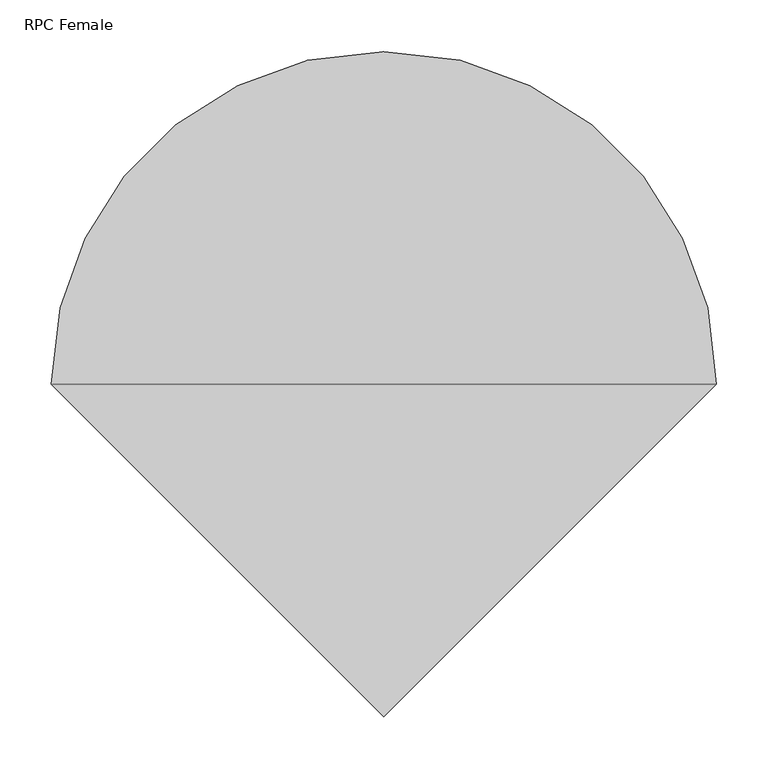
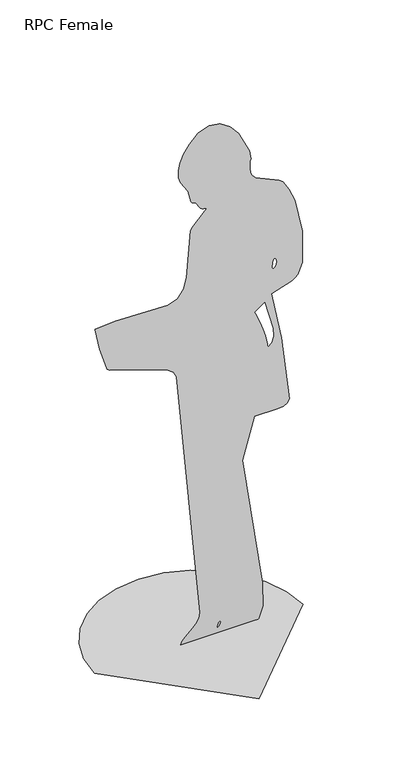
"""IFC4 building model written with IfcOpenShell, lengths in millimetres: proxy geometry, RPC Female : Lisa."""

import ifcopenshell
import ifcopenshell.guid

model = None  # the IFC model being written
_history = None  # IfcOwnerHistory: only IFC2X3 demands one
_inside = {}  # id of a spatial element -> (the spatial element, [elements in it])
_under = {}  # id of a project, library or spatial element -> (it, [spatial elements below it])
_declared = {}  # id of a project -> (the project, [libraries it declares])
_typed = {}  # id of a type object -> (the type object, [elements of that type])
_made_of = {}  # id of a material, layer set ... -> (it, [elements and type objects made of it])


def new_model(schema):
    """Start an empty IFC model of exactly this schema.

    Asked for "IFC4X3", IfcOpenShell would pick the latest addendum, in which some entities
    have other attributes; the version numbers below select the first issue.
    IFC2X3 requires an IfcOwnerHistory on every rooted entity: one is made here for all.
    """
    global model, _history
    if schema == "IFC4X3":
        model = ifcopenshell.file(schema_version=(4, 3, 0, 0))
    else:
        model = ifcopenshell.file(schema=schema)
    _inside.clear()
    _under.clear()
    _declared.clear()
    _typed.clear()
    _made_of.clear()
    _history = None
    if model.schema == "IFC2X3":
        org = make("IfcOrganization", Name="unknown")
        user = make(
            "IfcPersonAndOrganization",
            ThePerson=make("IfcPerson", FamilyName="unknown"),
            TheOrganization=org,
        )
        app = make(
            "IfcApplication",
            ApplicationDeveloper=org,
            Version="unknown",
            ApplicationFullName="unknown",
            ApplicationIdentifier="unknown",
        )
        _history = make(
            "IfcOwnerHistory",
            OwningUser=user,
            OwningApplication=app,
            ChangeAction="ADDED",
            CreationDate=0,
        )
    return model


def make(cls, **values):
    """One entity of the class cls with the attributes given. An attribute that is None is left unset."""
    return model.create_entity(
        cls, **{name: value for name, value in values.items() if value is not None}
    )


def rooted(cls, **values):
    """An entity with a GlobalId (a new one), such as an element, a storey or a relation."""
    return make(cls, GlobalId=ifcopenshell.guid.new(), OwnerHistory=_history, **values)


def si_unit(unit_type, name, prefix=None):
    """IfcSIUnit, for example si_unit("LENGTHUNIT", "METRE", prefix="MILLI")."""
    return make("IfcSIUnit", UnitType=unit_type, Prefix=prefix, Name=name)


def assignment(units):
    """IfcUnitAssignment: the units of a project."""
    return None if units is None else make("IfcUnitAssignment", Units=units)


def point(xyz):
    """IfcCartesianPoint."""
    return None if xyz is None else make("IfcCartesianPoint", Coordinates=xyz)


def direction(xyz):
    """IfcDirection."""
    return None if xyz is None else make("IfcDirection", DirectionRatios=xyz)


def frame(location, z_axis=None, x_axis=None):
    """IfcAxis2Placement3D, a coordinate frame: its origin and axes. An axis left out is left unset."""
    return make(
        "IfcAxis2Placement3D",
        Location=point(location),
        Axis=direction(z_axis),
        RefDirection=direction(x_axis),
    )


def origin():
    """The frame at (0, 0, 0) with its axes left unset."""
    return frame((0.0, 0.0, 0.0))


def place(relative_to, where):
    """IfcLocalPlacement: puts the frame where relative to a parent placement (None: the world)."""
    return make(
        "IfcLocalPlacement", PlacementRelTo=relative_to, RelativePlacement=where
    )


def context(
    kind, dimensions, precision=None, world=None, true_north=None, identifier=None
):
    """IfcGeometricRepresentationContext, for example the 3D "Model" context."""
    return make(
        "IfcGeometricRepresentationContext",
        ContextIdentifier=identifier,
        ContextType=kind,
        CoordinateSpaceDimension=dimensions,
        Precision=precision,
        WorldCoordinateSystem=world,
        TrueNorth=true_north,
    )


def project(units=None, contexts=None):
    """IfcProject with its units and contexts."""
    return rooted(
        "IfcProject",
        Name="project",
        RepresentationContexts=contexts,
        UnitsInContext=assignment(units),
    )


def spatial(cls, under=None, at=None, **own):
    """A site, building, storey or space (cls), placed at a placement, below another one or the project."""
    s = rooted(cls, ObjectPlacement=at, **own)
    if under is not None:
        _under.setdefault(under.id(), (under, []))[1].append(s)
    return s


def point_list(points):
    """IfcCartesianPointList2D or 3D."""
    cls = (
        "IfcCartesianPointList2D" if len(points[0]) == 2 else "IfcCartesianPointList3D"
    )
    return make(cls, CoordList=points)


def triangles(points, corners, closed=None, point_numbers=None):
    """IfcTriangulatedFaceSet: each triangle names its three corners, points numbered from 1."""
    return make(
        "IfcTriangulatedFaceSet",
        Coordinates=point_list(points),
        Closed=closed,
        CoordIndex=corners,
        PnIndex=point_numbers,
    )


def shape(context_of_items, identifier, shape_type, items):
    """IfcShapeRepresentation: the items that make up one representation, for example the "Body"."""
    return make(
        "IfcShapeRepresentation",
        ContextOfItems=context_of_items,
        RepresentationIdentifier=identifier,
        RepresentationType=shape_type,
        Items=items,
    )


def source(mapping_origin, context_of_items, identifier, shape_type, items):
    """IfcRepresentationMap: a shape defined once, which mapped items show again and again."""
    return make(
        "IfcRepresentationMap",
        MappingOrigin=mapping_origin,
        MappedRepresentation=shape(context_of_items, identifier, shape_type, items),
    )


def transform(
    local_origin,
    x_axis=None,
    y_axis=None,
    z_axis=None,
    scale=None,
    scale2=None,
    scale3=None,
    uniform=True,
):
    """IfcCartesianTransformationOperator3D, or its non-uniform kind. x_axis, y_axis, z_axis: its Axis1, 2, 3."""
    if uniform:
        return make(
            "IfcCartesianTransformationOperator3D",
            Axis1=direction(x_axis),
            Axis2=direction(y_axis),
            LocalOrigin=point(local_origin),
            Scale=scale,
            Axis3=direction(z_axis),
        )
    return make(
        "IfcCartesianTransformationOperator3DnonUniform",
        Axis1=direction(x_axis),
        Axis2=direction(y_axis),
        LocalOrigin=point(local_origin),
        Scale=scale,
        Axis3=direction(z_axis),
        Scale2=scale2,
        Scale3=scale3,
    )


def mapped(mapping_source, mapping_target):
    """IfcMappedItem: shows the shape of a source again, moved by a transform."""
    return make(
        "IfcMappedItem", MappingSource=mapping_source, MappingTarget=mapping_target
    )


def made_of(thing, what):
    """Note that an element or type object is made of a material, layer set ...; save() writes the relation."""
    if what is not None:
        _made_of.setdefault(what.id(), (what, []))[1].append(thing)
    return thing


def element(
    cls,
    number,
    at=None,
    inside=None,
    cuts=None,
    type_object=None,
    material=None,
    context=None,
    identifier="Body",
    shape_type=None,
    held_by="IfcProductDefinitionShape",
    body=None,
    shapes=None,
    **own,
):
    """One element of the class cls, such as IfcWall. Its Tag is "e" and its number.

    at: its placement. inside: the storey or other place that contains it. cuts: it is an
    opening in that element (IfcRelVoidsElement). A single representation is given by context,
    identifier, shape_type and body (its items); several are given by shapes. held_by: the class
    of the entity that holds the representations. save() writes the other relations.
    """
    e = rooted(cls, Tag="e%d" % number, ObjectPlacement=at, **own)
    if body is not None:
        shapes = [shape(context, identifier, shape_type, body)]
    if shapes is not None:
        e.Representation = make(held_by, Representations=shapes)
    if inside is not None:
        _inside.setdefault(inside.id(), (inside, []))[1].append(e)
    if cuts is not None:
        rooted(
            "IfcRelVoidsElement", RelatingBuildingElement=cuts, RelatedOpeningElement=e
        )
    if type_object is not None:
        _typed.setdefault(type_object.id(), (type_object, []))[1].append(e)
    return made_of(e, material)


def aggregate(whole, parts):
    """IfcRelAggregates: a whole, such as a stair, and the parts it consists of."""
    return rooted("IfcRelAggregates", RelatingObject=whole, RelatedObjects=parts)


def save(model, path):
    """Write the relations noted so far, then the file.

    IfcRelAggregates (storeys below a building ...), IfcRelContainedInSpatialStructure (elements
    in a storey), IfcRelDefinesByType, IfcRelAssociatesMaterial and IfcRelDeclares: one each for
    every whole, place, type object, material and project.
    """
    for whole, parts in _under.values():
        aggregate(whole, parts)
    for where, things in _inside.values():
        rooted(
            "IfcRelContainedInSpatialStructure",
            RelatedElements=things,
            RelatingStructure=where,
        )
    for kind, things in _typed.values():
        rooted("IfcRelDefinesByType", RelatedObjects=things, RelatingType=kind)
    for what, things in _made_of.values():
        rooted("IfcRelAssociatesMaterial", RelatedObjects=things, RelatingMaterial=what)
    for by, libraries in _declared.values():
        rooted("IfcRelDeclares", RelatingContext=by, RelatedDefinitions=libraries)
    model.write(path)


def rpc_female_aec5a013(model_context):
    return source(origin(), model_context, "Body", "Tessellation", [
        triangles([(323.55714, 0.0002011, 4.31e-05), (315.003338, 74.1380801, 4.31e-05), (290.6422523, 142.2218604, 4.31e-05), (252.4244724, 202.3008604, 4.31e-05), (202.3008059, 252.4245814, 4.31e-05), (142.2217514, 290.6422886, 4.31e-05), (74.1379711, 315.003447, 4.31e-05), (0.0001118, 323.557249, 4.31e-05), (-74.1377576, 315.003447, 4.31e-05), (-142.2215424, 290.6423431, 4.31e-05), (-202.3005515, 252.4245814, 4.31e-05), (-252.4243089, 202.3009149, 4.31e-05), (-290.6419797, 142.2218422, 4.31e-05), (-315.0031199, 74.1380664, 4.31e-05), (-323.556922, 0.0002066, 4.31e-05), (0.0001345, -323.556813, 4.31e-05), (239.7155461, -0.0024821, 1166.2291054), (241.5671591, -0.0024453, 1161.6157969), (242.5844117, -0.0023971, 1155.5697269), (242.4387992, -0.0023449, 1149.0417097), (240.802035, -0.0022965, 1142.9829952), (237.3454509, -0.0022592, 1138.3443249), (231.7406877, -0.0022408, 1136.0765854), (228.7156361, -0.0022542, 1137.7761183), (227.3342342, -0.0022926, 1142.5880339), (228.6198207, -0.0024031, 1156.4203291), (230.8453571, -0.0024548, 1162.8766211), (233.8316392, -0.0024904, 1167.3168297), (237.3580228, -0.0024998, 1168.4587658), (232.3851614, -0.0006708, 939.5053717), (233.2271703, -0.0004644, 913.6590569), (228.0144798, -0.0003049, 893.7186316), (214.8887911, -0.0002183, 882.9673256), (212.8489084, -0.0003717, 902.1807604), (207.5316821, -0.0005509, 924.6499557), (200.1408723, -0.0007392, 948.2795454), (191.8801301, -0.0009201, 970.9742357), (183.9532157, -0.0010767, 990.6387331), (177.563762, -0.0011925, 1005.1777439), (173.9154927, -0.0012508, 1012.4958292), (205.6367214, -0.0014424, 1036.2868189), (68.0155341, 0.0065606, 35.1859178), (68.3548802, 0.0065864, 31.9534865), (67.1147442, 0.0066181, 27.9900225), (62.1449576, 0.0066794, 20.3530545), (59.5397978, 0.0066989, 17.9209935), (57.6041283, 0.0067044, 17.2407831), (56.3838631, 0.0066925, 18.7385183), (56.501216, 0.0066679, 21.8255596), (59.4210051, 0.0066023, 30.0203991), (61.5595964, 0.0065723, 33.7551594), (63.7080572, 0.0065516, 36.3327024), (65.5344401, 0.0065457, 37.0666397), (199.6881201, 0.0065196, 39.4558675), (198.4421388, 0.0059101, 115.768188), (135.8335603, 0.0025305, 539.3201328), (174.0394677, 0.0014804, 670.542065), (245.5741638, 0.0014783, 670.3427313), (262.8130825, 0.0014526, 673.4447222), (275.84906, 0.0013998, 679.9665625), (282.7096696, 0.0013115, 690.9874741), (257.8416199, -0.0003504, 899.2227287), (226.66042, -0.0015969, 1055.4929867), (289.796737, -0.0017705, 1076.8137056), (300.5432649, -0.0018246, 1083.5191103), (308.4004706, -0.0018879, 1091.3857813), (322.1901449, -0.0021673, 1126.2816891), (322.886178, -0.0029802, 1228.0536747), (298.565951, -0.0038491, 1337.0047279), (281.0851866, -0.0041986, 1380.8742886), (262.2230204, -0.0044349, 1410.5811962), (250.0464744, -0.0045155, 1420.7485989), (176.8737423, -0.0047799, 1454.3395718), (165.8199294, -0.0048739, 1466.1760586), (162.904337, -0.00492, 1471.9682922), (160.6014253, -0.0049813, 1479.6591019), (159.0181643, -0.0050521, 1488.5277466), (159.6554438, -0.0052634, 1514.9892128), (162.0199978, -0.0053144, 1521.3580101), (157.2200546, -0.0055454, 1550.3042084), (123.1476431, -0.0060968, 1619.5682945), (96.7598279, -0.0063371, 1649.8205177), (66.0607524, -0.0065002, 1670.4420788), (32.4927251, -0.006546, 1676.4), (-2.5019012, -0.0064344, 1662.6614491), (-29.4130598, -0.0062285, 1637.0601048), (-47.9634423, -0.0060193, 1610.9874229), (-59.0861691, -0.0058139, 1585.3437847), (-63.7143613, -0.0056195, 1561.0297165), (-62.7811788, -0.0054432, 1538.9461807), (-57.2196996, -0.0052921, 1519.9931225), (-33.763421, -0.0050094, 1484.4516872), (-23.4502333, -0.0046956, 1445.0888283), (-21.9944378, -0.0046776, 1442.8234142), (-21.2605709, -0.0046685, 1441.6813328), (-20.7350171, -0.0046648, 1441.2126114), (-19.9041471, -0.0046628, 1440.9669868), (-18.2543602, -0.0046592, 1440.4947773), (-15.272017, -0.0046501, 1439.3457195), (-10.4435032, -0.0046322, 1437.069841), (5.6148508, -0.0044554, 1414.8345703), (9.271162, -0.0044304, 1411.6780769), (14.0533369, -0.0044149, 1409.7007267), (20.5959585, -0.0044097, 1409.0118153), (23.5075336, -0.0043928, 1406.8681961), (19.6093908, -0.004345, 1400.9185593), (-20.4444416, -0.0040148, 1359.8386539), (-25.6642197, -0.0039395, 1350.4428612), (-38.3351555, -0.0027409, 1200.4557953), (-47.8502179, -0.0024695, 1166.542749), (-65.8721511, -0.0022718, 1141.9037006), (-95.3849391, -0.0021789, 1130.4592684), (-259.8646069, -0.0022058, 1134.9048546), (-318.3029549, -0.00218, 1132.0589527), (-321.9124002, -0.0021697, 1130.793405), (-322.5551662, -0.0021658, 1130.3113123), (-322.88596, -0.0021617, 1129.7984076), (-308.628291, -0.0016091, 1060.5184067), (-285.0727521, -0.0010211, 986.743404), (-277.451851, -0.0009685, 980.1137941), (-100.0195944, -0.0004954, 919.7210415), (-78.3459718, -0.000372, 904.1187235), (-69.2809683, -0.0002246, 885.6107689), (3.4135975, 0.0061696, 84.5657866), (0.0373612, 0.0063051, 67.6165078), (-8.1503865, 0.0064193, 53.3745945), (-19.3216154, 0.0065172, 41.1892918), (-43.3023578, 0.0066846, 20.3858174), (-52.4557871, 0.0067643, 10.4659911), (-57.2805471, 0.0068482, 0.0), (186.0811745, 0.0068354, 0.0)], [[15, 16, 1], [14, 15, 1], [14, 1, 2], [13, 14, 2], [13, 2, 3], [13, 3, 4], [12, 13, 4], [11, 12, 4], [11, 4, 5], [11, 5, 6], [11, 6, 7], [11, 7, 8], [11, 8, 9], [11, 9, 10], [33, 56, 57], [39, 40, 53], [38, 39, 53], [37, 38, 53], [129, 130, 131], [128, 129, 131], [22, 23, 63], [33, 57, 58], [33, 58, 59], [33, 59, 60], [33, 60, 61], [33, 61, 62], [32, 33, 62], [31, 32, 62], [30, 31, 62], [41, 30, 62], [41, 62, 63], [22, 63, 64], [22, 64, 65], [22, 65, 66], [22, 66, 67], [21, 22, 67], [20, 21, 67], [19, 20, 67], [18, 19, 67], [18, 67, 68], [17, 18, 68], [29, 17, 68], [63, 23, 24], [52, 53, 40], [37, 53, 42], [29, 68, 69], [28, 29, 69], [41, 63, 24], [115, 116, 117], [114, 115, 117], [114, 117, 118], [113, 114, 118], [113, 118, 119], [113, 119, 120], [112, 113, 120], [112, 120, 121], [111, 112, 121], [111, 121, 122], [28, 69, 70], [28, 70, 71], [28, 71, 72], [28, 72, 73], [27, 28, 73], [40, 41, 24], [40, 24, 25], [51, 52, 40], [110, 111, 122], [110, 122, 123], [27, 73, 74], [83, 84, 85], [82, 83, 85], [82, 85, 86], [81, 82, 86], [81, 86, 87], [81, 87, 88], [81, 88, 89], [81, 89, 90], [81, 90, 91], [80, 81, 91], [80, 91, 92], [79, 80, 92], [78, 79, 92], [77, 78, 92], [77, 92, 93], [77, 93, 94], [77, 94, 95], [77, 95, 96], [77, 96, 97], [77, 97, 98], [77, 98, 99], [77, 99, 100], [76, 77, 100], [76, 100, 101], [76, 101, 102], [76, 102, 103], [76, 103, 104], [76, 104, 105], [75, 76, 105], [74, 75, 105], [27, 74, 105], [27, 105, 106], [27, 106, 107], [27, 107, 108], [27, 108, 109], [26, 27, 109], [25, 26, 109], [25, 109, 110], [25, 110, 123], [40, 25, 123], [51, 40, 123], [51, 123, 124], [51, 124, 125], [50, 51, 125], [50, 125, 126], [49, 50, 126], [49, 126, 127], [48, 49, 127], [48, 127, 128], [47, 48, 128], [47, 128, 131], [46, 47, 131], [45, 46, 131], [44, 45, 131], [43, 44, 131], [43, 131, 54], [43, 54, 55], [42, 43, 55], [56, 33, 34], [56, 34, 35], [56, 35, 36], [56, 36, 37], [56, 37, 42], [56, 42, 55]], closed=False),
    ])


if __name__ == "__main__":
    model = new_model("IFC4")
    model_context = context("Model", 3, world=origin())
    ifc_project = project(units=[si_unit("LENGTHUNIT", "METRE", prefix="MILLI")], contexts=[model_context])
    site = spatial("IfcSite", under=ifc_project)
    building = spatial("IfcBuilding", under=site)
    placement = place(None, origin())
    rpc_female_shape = rpc_female_aec5a013(model_context)
    element("IfcBuildingElementProxy", 1, Name="RPC Female : Lisa", ObjectType="RPC Female : Lisa", at=placement, inside=building, context=model_context, shape_type="MappedRepresentation", body=[
        mapped(rpc_female_shape, transform((0.0, 0.0, 0.0), x_axis=(1.0, 0.0, 0.0), y_axis=(0.0, 1.0, 0.0), z_axis=(0.0, 0.0, 1.0))),
    ])
    save(model, "model.ifc")

# Revit data of these elements
# Type "RPC Female : Lisa"
#   built-in parameter 1005198 = "{2, 15},{22, RPC-8-N2L1-0HXP-BER1-C},{1, 0},{1, 0},{2, 23},{1, 8},{5, Color},{1, 0},{1, 0},{3, 0.8},{3, 0.8},{3, 0.8},{1, 8},{7, BBoxMin},{1, 0},{1, 0},{1, 0},{1, 0},{1, 0},{1, 8},{7, BBoxMax},{1, 0},{1, 0},{1, 0},{1, 0},{1, 0},{2, 11},{9, RPCTypeId},{1, 0},{1, 0},{22, RPC-8-N2L1-0HXP-BER1-C},{1, 6},{14, RPCPlantHeight},{1, 0},{1, 0},{3, 5.5},{2, 11},{7, keyword},{1, 0},{1, 0},{34, :RPCs:People [Casual]:Geometry:RPC},{2, 11},{8, category},{1, 0},{1, 0},{15, People [Casual]},{2, 11},{12, LocalizedUID},{1, 0},{1, 0},{14, Lisa (1/2 res)},{2, 14},{6, Height},{1, 0},{1, 0},{3, 5.5},{1, 2},{16, Cast Reflections},{1, 0},{1, 0},{1, 0},{1, 2},{6, Jitter},{1, 0},{1, 0},{1, 0},{1, 2},{9, Billboard},{1, 0},{1, 0},{1, 0},{1, 2},{12, Cast Shadows},{1, 0},{1, 0},{1, 1},{1, 2},{20, Apply Filter Effects},{1, 0},{1, 0},{1, 0},{2, 11},{28, Apply Filter Effects-Text-FC},{1, 0},{1, 0},{4, None},{1, 2},{5, Cycle},{1, 0},{1, 0},{1, 1},{1, 4},{17, Cycle Start Frame},{1, 0},{1, 0},{1, 0},{1, 2},{9, Ping Pong},{1, 0},{1, 0},{1, 0},{1, 4},{21, Ping Pong Begin Frame},{1, 0},{1, 0},{1, 0},{1, 4},{21, Ping Pong Start Frame},{1, 0},{1, 0},{1, 0},{1, 4},{19, Ping Pong End Frame},{1, 0},{1, 0},{3, 599},{1, 2},{19, Use Specified Frame},{1, 0},{1, 0},{1, 0},{1, 4},{13, Current Frame},{1, 0},{1, 0},{1, 0},{21, assetlibrary_base.fbx},{1, 5},"
#   built-in parameter 1005195 = "RPC-8-N2L1-0HXP-BER1-C"
#   Height = 0
